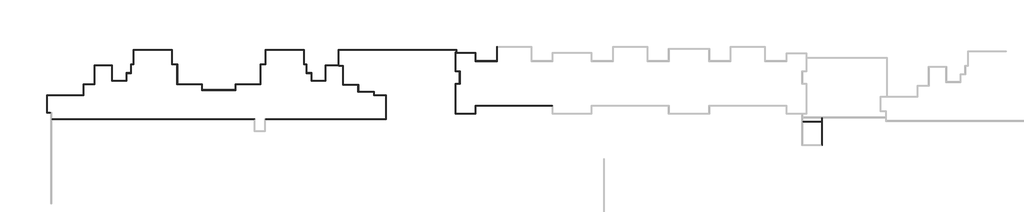
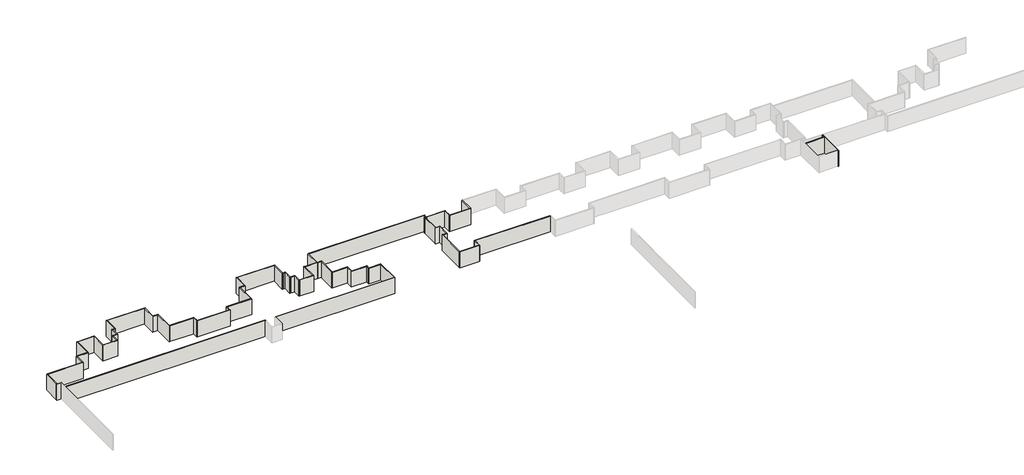
# One storey, part 5 of 8: 63 walls.
"""IFC4 building model written with IfcOpenShell, lengths in millimetres."""

from ifc_helpers import new_model, si_unit, origin, origin_with_axes, place, context, project, spatial, polyline, outline, extrude, faceted_brep, element, save

model = new_model("IFC4")

# Units and contexts
model_context = context("Model", 3, world=origin())
ifc_project = project(units=[si_unit("LENGTHUNIT", "METRE", prefix="MILLI")], contexts=[model_context])

# Site, building, storey
site = spatial("IfcSite", under=ifc_project)
building = spatial("IfcBuilding", under=site)
storey = spatial("IfcBuildingStorey", under=building, Name="户型图", Elevation=0.0)

# Walls
placement = place(None, origin())
element("IfcWall", 1, ObjectType="所有墙体", at=placement, inside=storey, context=model_context, shape_type="Brep", body=[
    faceted_brep([(84990.3013454, 129402.6292795, 0.0), (84259.8101643, 129402.6292795, 0.0), (84139.8101643, 129402.6292795, 0.0), (84139.8101643, 129402.6292795, 3300.0), (84259.8101643, 129402.6292795, 3300.0), (84990.3013454, 129402.6292795, 3300.0), (84990.3013454, 129282.6292795, 0.0), (84990.3013454, 129282.6292795, 3300.0), (84139.8101643, 129282.6292795, 3300.0), (84139.8101643, 129282.6292795, 0.0)], [[[0, 1, 2, 3, 4, 5]], [[6, 7, 8, 9]], [[2, 1, 0, 6, 9]], [[5, 4, 3, 8, 7]], [[0, 5, 7, 6]], [[3, 2, 9, 8]]]),
])
element("IfcWall", 2, ObjectType="所有墙体", at=placement, inside=storey, context=model_context, shape_type="Brep", body=[
    faceted_brep([(84259.8101643, 129402.6292795, 0.0), (84259.8101643, 132682.6292767, 0.0), (84259.8101643, 132802.6292767, 0.0), (84259.8101643, 132802.6292767, 3300.0), (84259.8101643, 132682.6292767, 3300.0), (84259.8101643, 129402.6292795, 3300.0), (84139.8101643, 129402.6292795, 0.0), (84139.8101643, 129402.6292795, 3300.0), (84139.8101643, 132802.6292767, 3300.0), (84139.8101643, 132802.6292767, 0.0)], [[[0, 1, 2, 3, 4, 5]], [[6, 7, 8, 9]], [[2, 1, 0, 6, 9]], [[5, 4, 3, 8, 7]], [[0, 5, 7, 6]], [[3, 2, 9, 8]]]),
])
element("IfcWall", 3, ObjectType="所有墙体", at=placement, inside=storey, context=model_context, shape_type="Brep", body=[
    faceted_brep([(84259.8101643, 132682.6292767, 0.0), (91359.8101643, 132682.6292767, 0.0), (91359.8101643, 132682.6292767, 3300.0), (84259.8101643, 132682.6292767, 3300.0), (84259.8101643, 132802.6292767, 0.0), (84259.8101643, 132802.6292767, 3300.0), (91239.8101643, 132802.6292767, 3300.0), (91359.8101643, 132802.6292767, 3300.0), (91359.8101643, 132802.6292767, 0.0), (91239.8101643, 132802.6292767, 0.0)], [[[0, 1, 2, 3]], [[4, 5, 6, 7, 8, 9]], [[1, 0, 4, 9, 8]], [[3, 2, 7, 6, 5]], [[0, 3, 5, 4]], [[2, 1, 8, 7]]]),
])
element("IfcWall", 4, ObjectType="所有墙体", at=placement, inside=storey, context=model_context, shape_type="Brep", body=[
    faceted_brep([(91359.8101643, 132802.6292767, 0.0), (91359.8101643, 134782.6292766, 0.0), (91359.8101643, 134902.6292766, 0.0), (91359.8101643, 134902.6292766, 3300.0), (91359.8101643, 134782.6292766, 3300.0), (91359.8101643, 132802.6292767, 3300.0), (91239.8101643, 132802.6292767, 0.0), (91239.8101643, 132802.6292767, 3300.0), (91239.8101643, 134902.6292766, 3300.0), (91239.8101643, 134902.6292766, 0.0)], [[[0, 1, 2, 3, 4, 5]], [[6, 7, 8, 9]], [[2, 1, 0, 6, 9]], [[5, 4, 3, 8, 7]], [[0, 5, 7, 6]], [[3, 2, 9, 8]]]),
])
element("IfcWall", 5, ObjectType="所有墙体", at=placement, inside=storey, context=model_context, shape_type="Brep", body=[
    faceted_brep([(91359.8101643, 134782.6292766, 0.0), (93559.8101642, 134782.6292766, 0.0), (93559.8101642, 134782.6292766, 3300.0), (91359.8101643, 134782.6292766, 3300.0), (91359.8101643, 134902.6292766, 0.0), (91359.8101643, 134902.6292766, 3300.0), (93439.8101642, 134902.6292766, 3300.0), (93559.8101642, 134902.6292766, 3300.0), (93559.8101642, 134902.6292766, 0.0), (93439.8101642, 134902.6292766, 0.0)], [[[0, 1, 2, 3]], [[4, 5, 6, 7, 8, 9]], [[1, 0, 4, 9, 8]], [[3, 2, 7, 6, 5]], [[0, 3, 5, 4]], [[2, 1, 8, 7]]]),
])
element("IfcWall", 6, ObjectType="所有墙体", at=placement, inside=storey, context=model_context, shape_type="Brep", body=[
    faceted_brep([(93559.8101642, 134902.6292766, 0.0), (93559.8101642, 138482.6292767, 0.0), (93559.8101642, 138602.6292767, 0.0), (93559.8101642, 138602.6292767, 3300.0), (93559.8101642, 138482.6292767, 3300.0), (93559.8101642, 134902.6292766, 3300.0), (93439.8101642, 134902.6292766, 0.0), (93439.8101642, 134902.6292766, 3300.0), (93439.8101642, 138602.6292767, 3300.0), (93439.8101642, 138602.6292767, 0.0)], [[[0, 1, 2, 3, 4, 5]], [[6, 7, 8, 9]], [[2, 1, 0, 6, 9]], [[5, 4, 3, 8, 7]], [[0, 5, 7, 6]], [[3, 2, 9, 8]]]),
])
element("IfcWall", 7, ObjectType="所有墙体", at=placement, inside=storey, context=model_context, shape_type="Brep", body=[
    faceted_brep([(93559.8101642, 138482.6292767, 0.0), (96839.8101642, 138482.6292767, 0.0), (96959.8101642, 138482.6292767, 0.0), (96959.8101642, 138482.6292767, 3300.0), (96839.8101642, 138482.6292767, 3300.0), (93559.8101642, 138482.6292767, 3300.0), (93559.8101642, 138602.6292767, 0.0), (93559.8101642, 138602.6292767, 3300.0), (96959.8101642, 138602.6292767, 3300.0), (96959.8101642, 138602.6292767, 0.0)], [[[0, 1, 2, 3, 4, 5]], [[6, 7, 8, 9]], [[2, 1, 0, 6, 9]], [[5, 4, 3, 8, 7]], [[0, 5, 7, 6]], [[3, 2, 9, 8]]]),
])
element("IfcWall", 8, ObjectType="所有墙体", at=placement, inside=storey, context=model_context, shape_type="Brep", body=[
    faceted_brep([(96839.8101642, 138482.6292767, 0.0), (96839.8101642, 135482.6292767, 0.0), (96839.8101642, 135482.6292767, 3300.0), (96839.8101642, 138482.6292767, 3300.0), (96959.8101642, 138482.6292767, 0.0), (96959.8101642, 138482.6292767, 3300.0), (96959.8101642, 135602.6292767, 3300.0), (96959.8101642, 135482.6292767, 3300.0), (96959.8101642, 135482.6292767, 0.0), (96959.8101642, 135602.6292767, 0.0)], [[[0, 1, 2, 3]], [[4, 5, 6, 7, 8, 9]], [[1, 0, 4, 9, 8]], [[3, 2, 7, 6, 5]], [[0, 3, 5, 4]], [[2, 1, 8, 7]]]),
])
element("IfcWall", 9, ObjectType="所有墙体", at=placement, inside=storey, context=model_context, shape_type="Brep", body=[
    faceted_brep([(96959.8101642, 135482.6292767, 0.0), (99760.1109232, 135482.6292767, 0.0), (99760.1109232, 135482.6292767, 3300.0), (96959.8101642, 135482.6292767, 3300.0), (96959.8101642, 135602.6292767, 0.0), (96959.8101642, 135602.6292767, 3300.0), (99640.1109232, 135602.6292767, 3300.0), (99760.1109232, 135602.6292767, 3300.0), (99760.1109232, 135602.6292767, 0.0), (99640.1109232, 135602.6292767, 0.0)], [[[0, 1, 2, 3]], [[4, 5, 6, 7, 8, 9]], [[1, 0, 4, 9, 8]], [[3, 2, 7, 6, 5]], [[0, 3, 5, 4]], [[2, 1, 8, 7]]]),
])
element("IfcWall", 10, ObjectType="所有墙体", at=placement, inside=storey, context=model_context, shape_type="Brep", body=[
    faceted_brep([(99760.1109232, 135602.6292767, 0.0), (99760.1109232, 136982.6292752, 0.0), (99760.1109232, 137102.6292752, 0.0), (99760.1109232, 137102.6292752, 3300.0), (99760.1109232, 136982.6292752, 3300.0), (99760.1109232, 135602.6292767, 3300.0), (99640.1109232, 135602.6292767, 0.0), (99640.1109232, 135602.6292767, 3300.0), (99640.1109232, 137102.6292752, 3300.0), (99640.1109232, 137102.6292752, 0.0)], [[[0, 1, 2, 3, 4, 5]], [[6, 7, 8, 9]], [[2, 1, 0, 6, 9]], [[5, 4, 3, 8, 7]], [[0, 5, 7, 6]], [[3, 2, 9, 8]]]),
])
element("IfcWall", 11, ObjectType="所有墙体", at=placement, inside=storey, context=model_context, shape_type="Brep", body=[
    faceted_brep([(99760.1109232, 136982.6292752, 0.0), (100659.8101643, 136982.6292752, 0.0), (100659.8101643, 136982.6292752, 3300.0), (99760.1109232, 136982.6292752, 3300.0), (99760.1109232, 137102.6292752, 0.0), (99760.1109232, 137102.6292752, 3300.0), (100539.8101643, 137102.6292752, 3300.0), (100659.8101643, 137102.6292752, 3300.0), (100659.8101643, 137102.6292752, 0.0), (100539.8101643, 137102.6292752, 0.0)], [[[0, 1, 2, 3]], [[4, 5, 6, 7, 8, 9]], [[1, 0, 4, 9, 8]], [[3, 2, 7, 6, 5]], [[0, 3, 5, 4]], [[2, 1, 8, 7]]]),
])
element("IfcWall", 12, ObjectType="所有墙体", at=placement, inside=storey, context=model_context, shape_type="Brep", body=[
    faceted_brep([(100659.8101643, 137102.6292752, 0.0), (100659.8101643, 138682.6292768, 0.0), (100659.8101643, 138802.6292768, 0.0), (100659.8101643, 138802.6292768, 3300.0), (100659.8101643, 138682.6292768, 3300.0), (100659.8101643, 137102.6292752, 3300.0), (100539.8101643, 137102.6292752, 0.0), (100539.8101643, 137102.6292752, 3300.0), (100539.8101643, 138802.6292768, 3300.0), (100539.8101643, 138802.6292768, 0.0)], [[[0, 1, 2, 3, 4, 5]], [[6, 7, 8, 9]], [[2, 1, 0, 6, 9]], [[5, 4, 3, 8, 7]], [[0, 5, 7, 6]], [[3, 2, 9, 8]]]),
])
element("IfcWall", 13, ObjectType="所有墙体", at=placement, inside=storey, context=model_context, shape_type="Brep", body=[
    faceted_brep([(100659.8101643, 138682.6292768, 0.0), (101159.8101643, 138682.6292768, 0.0), (101159.8101643, 138682.6292768, 3300.0), (100659.8101643, 138682.6292768, 3300.0), (100659.8101643, 138802.6292768, 0.0), (100659.8101643, 138802.6292768, 3300.0), (101039.8101643, 138802.6292768, 3300.0), (101159.8101643, 138802.6292768, 3300.0), (101159.8101643, 138802.6292768, 0.0), (101039.8101643, 138802.6292768, 0.0)], [[[0, 1, 2, 3]], [[4, 5, 6, 7, 8, 9]], [[1, 0, 4, 9, 8]], [[3, 2, 7, 6, 5]], [[0, 3, 5, 4]], [[2, 1, 8, 7]]]),
])
element("IfcWall", 14, ObjectType="所有墙体", at=placement, inside=storey, context=model_context, shape_type="Brep", body=[
    faceted_brep([(101159.8101643, 138802.6292768, 0.0), (101159.8101643, 141482.6292767, 0.0), (101159.8101643, 141602.6292767, 0.0), (101159.8101643, 141602.6292767, 3300.0), (101159.8101643, 141482.6292767, 3300.0), (101159.8101643, 138802.6292768, 3300.0), (101039.8101643, 138802.6292768, 0.0), (101039.8101643, 138802.6292768, 3300.0), (101039.8101643, 141602.6292767, 3300.0), (101039.8101643, 141602.6292767, 0.0)], [[[0, 1, 2, 3, 4, 5]], [[6, 7, 8, 9]], [[2, 1, 0, 6, 9]], [[5, 4, 3, 8, 7]], [[0, 5, 7, 6]], [[3, 2, 9, 8]]]),
])
element("IfcWall", 15, ObjectType="所有墙体", at=placement, inside=storey, context=model_context, shape_type="Brep", body=[
    faceted_brep([(101159.8101643, 141482.6292767, 0.0), (108539.8101642, 141482.6292767, 0.0), (108659.8101642, 141482.6292767, 0.0), (108659.8101642, 141482.6292767, 3300.0), (108539.8101642, 141482.6292767, 3300.0), (101159.8101643, 141482.6292767, 3300.0), (101159.8101643, 141602.6292767, 0.0), (101159.8101643, 141602.6292767, 3300.0), (108659.8101642, 141602.6292767, 3300.0), (108659.8101642, 141602.6292767, 0.0)], [[[0, 1, 2, 3, 4, 5]], [[6, 7, 8, 9]], [[2, 1, 0, 6, 9]], [[5, 4, 3, 8, 7]], [[0, 5, 7, 6]], [[3, 2, 9, 8]]]),
])
element("IfcWall", 16, ObjectType="所有墙体", at=placement, inside=storey, context=model_context, shape_type="Brep", body=[
    faceted_brep([(108539.8101642, 141482.6292767, 0.0), (108539.8101642, 138682.6292768, 0.0), (108539.8101642, 138682.6292768, 3300.0), (108539.8101642, 141482.6292767, 3300.0), (108659.8101642, 141482.6292767, 0.0), (108659.8101642, 141482.6292767, 3300.0), (108659.8101642, 138802.6292768, 3300.0), (108659.8101642, 138682.6292768, 3300.0), (108659.8101642, 138682.6292768, 0.0), (108659.8101642, 138802.6292768, 0.0)], [[[0, 1, 2, 3]], [[4, 5, 6, 7, 8, 9]], [[1, 0, 4, 9, 8]], [[3, 2, 7, 6, 5]], [[0, 3, 5, 4]], [[2, 1, 8, 7]]]),
])
element("IfcWall", 17, ObjectType="所有墙体", at=placement, inside=storey, context=model_context, shape_type="Brep", body=[
    faceted_brep([(108659.8101642, 138682.6292768, 0.0), (109539.8775938, 138682.6292768, 0.0), (109659.8775938, 138682.6292768, 0.0), (109659.8775938, 138682.6292768, 3300.0), (109539.8775938, 138682.6292768, 3300.0), (108659.8101642, 138682.6292768, 3300.0), (108659.8101642, 138802.6292768, 0.0), (108659.8101642, 138802.6292768, 3300.0), (109659.8775938, 138802.6292768, 3300.0), (109659.8775938, 138802.6292768, 0.0)], [[[0, 1, 2, 3, 4, 5]], [[6, 7, 8, 9]], [[2, 1, 0, 6, 9]], [[5, 4, 3, 8, 7]], [[0, 5, 7, 6]], [[3, 2, 9, 8]]]),
])
element("IfcWall", 18, ObjectType="所有墙体", at=placement, inside=storey, context=model_context, shape_type="Brep", body=[
    faceted_brep([(109539.8775938, 138682.6292768, 0.0), (109539.8775938, 134782.6292766, 0.0), (109539.8775938, 134782.6292766, 3300.0), (109539.8775938, 138682.6292768, 3300.0), (109659.8775938, 138682.6292768, 0.0), (109659.8775938, 138682.6292768, 3300.0), (109659.8775938, 134902.6292766, 3300.0), (109659.8775938, 134782.6292766, 3300.0), (109659.8775938, 134782.6292766, 0.0), (109659.8775938, 134902.6292766, 0.0)], [[[0, 1, 2, 3]], [[4, 5, 6, 7, 8, 9]], [[1, 0, 4, 9, 8]], [[3, 2, 7, 6, 5]], [[0, 3, 5, 4]], [[2, 1, 8, 7]]]),
])
element("IfcWall", 19, ObjectType="所有墙体", at=placement, inside=storey, context=model_context, shape_type="Brep", body=[
    faceted_brep([(109659.8775938, 134782.6292766, 0.0), (114389.8101643, 134782.6292766, 0.0), (114509.8101643, 134782.6292766, 0.0), (114509.8101643, 134782.6292766, 3300.0), (114389.8101643, 134782.6292766, 3300.0), (109659.8775938, 134782.6292766, 3300.0), (109659.8775938, 134902.6292766, 0.0), (109659.8775938, 134902.6292766, 3300.0), (114509.8101643, 134902.6292766, 3300.0), (114509.8101643, 134902.6292766, 0.0)], [[[0, 1, 2, 3, 4, 5]], [[6, 7, 8, 9]], [[2, 1, 0, 6, 9]], [[5, 4, 3, 8, 7]], [[0, 5, 7, 6]], [[3, 2, 9, 8]]]),
])
element("IfcWall", 20, ObjectType="所有墙体", at=placement, inside=storey, context=model_context, shape_type="Brep", body=[
    faceted_brep([(114389.8101643, 134782.6292766, 0.0), (114389.8101643, 133682.6292771, 0.0), (114389.8101643, 133682.6292771, 3300.0), (114389.8101643, 134782.6292766, 3300.0), (114509.8101643, 134782.6292766, 0.0), (114509.8101643, 134782.6292766, 3300.0), (114509.8101643, 133802.6292771, 3300.0), (114509.8101643, 133682.6292771, 3300.0), (114509.8101643, 133682.6292771, 0.0), (114509.8101643, 133802.6292771, 0.0)], [[[0, 1, 2, 3]], [[4, 5, 6, 7, 8, 9]], [[1, 0, 4, 9, 8]], [[3, 2, 7, 6, 5]], [[0, 3, 5, 4]], [[2, 1, 8, 7]]]),
])
element("IfcWall", 21, ObjectType="所有墙体", at=placement, inside=storey, context=model_context, shape_type="Brep", body=[
    faceted_brep([(114509.8101643, 133682.6292771, 0.0), (121009.8101642, 133682.6292771, 0.0), (121009.8101642, 133682.6292771, 3300.0), (114509.8101643, 133682.6292771, 3300.0), (114509.8101643, 133802.6292771, 0.0), (114509.8101643, 133802.6292771, 3300.0), (120889.8101642, 133802.6292771, 3300.0), (121009.8101642, 133802.6292771, 3300.0), (121009.8101642, 133802.6292771, 0.0), (120889.8101642, 133802.6292771, 0.0)], [[[0, 1, 2, 3]], [[4, 5, 6, 7, 8, 9]], [[1, 0, 4, 9, 8]], [[3, 2, 7, 6, 5]], [[0, 3, 5, 4]], [[2, 1, 8, 7]]]),
])
element("IfcWall", 22, ObjectType="所有墙体", at=placement, inside=storey, context=model_context, shape_type="Brep", body=[
    faceted_brep([(121009.8101642, 133802.6292771, 0.0), (121009.8101642, 134782.6292766, 0.0), (121009.8101642, 134902.6292766, 0.0), (121009.8101642, 134902.6292766, 3300.0), (121009.8101642, 134782.6292766, 3300.0), (121009.8101642, 133802.6292771, 3300.0), (120889.8101642, 133802.6292771, 0.0), (120889.8101642, 133802.6292771, 3300.0), (120889.8101642, 134902.6292766, 3300.0), (120889.8101642, 134902.6292766, 0.0)], [[[0, 1, 2, 3, 4, 5]], [[6, 7, 8, 9]], [[2, 1, 0, 6, 9]], [[5, 4, 3, 8, 7]], [[0, 5, 7, 6]], [[3, 2, 9, 8]]]),
])
element("IfcWall", 23, ObjectType="所有墙体", at=placement, inside=storey, context=model_context, shape_type="Brep", body=[
    faceted_brep([(121009.8101642, 134782.6292766, 0.0), (125856.9756647, 134782.6292766, 0.0), (125856.9756647, 134782.6292766, 3300.0), (121009.8101642, 134782.6292766, 3300.0), (121009.8101642, 134902.6292766, 0.0), (121009.8101642, 134902.6292766, 3300.0), (125736.9756647, 134902.6292766, 3300.0), (125856.9756647, 134902.6292766, 3300.0), (125856.9756647, 134902.6292766, 0.0), (125736.9756647, 134902.6292766, 0.0)], [[[0, 1, 2, 3]], [[4, 5, 6, 7, 8, 9]], [[1, 0, 4, 9, 8]], [[3, 2, 7, 6, 5]], [[0, 3, 5, 4]], [[2, 1, 8, 7]]]),
])
element("IfcWall", 24, ObjectType="所有墙体", at=placement, inside=storey, context=model_context, shape_type="Brep", body=[
    faceted_brep([(125856.9756647, 134902.6292766, 0.0), (125856.9756647, 138682.6292768, 0.0), (125856.9756647, 138802.6292768, 0.0), (125856.9756647, 138802.6292768, 3300.0), (125856.9756647, 138682.6292768, 3300.0), (125856.9756647, 134902.6292766, 3300.0), (125736.9756647, 134902.6292766, 0.0), (125736.9756647, 134902.6292766, 3300.0), (125736.9756647, 138802.6292768, 3300.0), (125736.9756647, 138802.6292768, 0.0)], [[[0, 1, 2, 3, 4, 5]], [[6, 7, 8, 9]], [[2, 1, 0, 6, 9]], [[5, 4, 3, 8, 7]], [[0, 5, 7, 6]], [[3, 2, 9, 8]]]),
])
element("IfcWall", 25, ObjectType="所有墙体", at=placement, inside=storey, context=model_context, shape_type="Brep", body=[
    faceted_brep([(125856.9756647, 138682.6292768, 0.0), (126856.9756647, 138682.6292768, 0.0), (126856.9756647, 138682.6292768, 3300.0), (125856.9756647, 138682.6292768, 3300.0), (125856.9756647, 138802.6292768, 0.0), (125856.9756647, 138802.6292768, 3300.0), (126736.9756647, 138802.6292768, 3300.0), (126856.9756647, 138802.6292768, 3300.0), (126856.9756647, 138802.6292768, 0.0), (126736.9756647, 138802.6292768, 0.0)], [[[0, 1, 2, 3]], [[4, 5, 6, 7, 8, 9]], [[1, 0, 4, 9, 8]], [[3, 2, 7, 6, 5]], [[0, 3, 5, 4]], [[2, 1, 8, 7]]]),
])
element("IfcWall", 26, ObjectType="所有墙体", at=placement, inside=storey, context=model_context, shape_type="Brep", body=[
    faceted_brep([(126856.9756647, 138802.6292768, 0.0), (126856.9756647, 141482.6292767, 0.0), (126856.9756647, 141602.6292767, 0.0), (126856.9756647, 141602.6292767, 3300.0), (126856.9756647, 141482.6292767, 3300.0), (126856.9756647, 138802.6292768, 3300.0), (126736.9756647, 138802.6292768, 0.0), (126736.9756647, 138802.6292768, 3300.0), (126736.9756647, 141602.6292767, 3300.0), (126736.9756647, 141602.6292767, 0.0)], [[[0, 1, 2, 3, 4, 5]], [[6, 7, 8, 9]], [[2, 1, 0, 6, 9]], [[5, 4, 3, 8, 7]], [[0, 5, 7, 6]], [[3, 2, 9, 8]]]),
])
element("IfcWall", 27, ObjectType="所有墙体", at=placement, inside=storey, context=model_context, shape_type="Brep", body=[
    faceted_brep([(126856.9756647, 141482.6292767, 0.0), (134239.8101637, 141482.6292767, 0.0), (134359.8101637, 141482.6292767, 0.0), (134359.8101637, 141482.6292767, 3300.0), (134239.8101637, 141482.6292767, 3300.0), (126856.9756647, 141482.6292767, 3300.0), (126856.9756647, 141602.6292767, 0.0), (126856.9756647, 141602.6292767, 3300.0), (134359.8101637, 141602.6292767, 3300.0), (134359.8101637, 141602.6292767, 0.0)], [[[0, 1, 2, 3, 4, 5]], [[6, 7, 8, 9]], [[2, 1, 0, 6, 9]], [[5, 4, 3, 8, 7]], [[0, 5, 7, 6]], [[3, 2, 9, 8]]]),
])
element("IfcWall", 28, ObjectType="所有墙体", at=placement, inside=storey, context=model_context, shape_type="Brep", body=[
    faceted_brep([(134239.8101637, 141482.6292767, 0.0), (134239.8101637, 138682.6292768, 0.0), (134239.8101637, 138682.6292768, 3300.0), (134239.8101637, 141482.6292767, 3300.0), (134359.8101637, 141482.6292767, 0.0), (134359.8101637, 141482.6292767, 3300.0), (134359.8101637, 138802.6292768, 3300.0), (134359.8101637, 138682.6292768, 3300.0), (134359.8101637, 138682.6292768, 0.0), (134359.8101637, 138802.6292768, 0.0)], [[[0, 1, 2, 3]], [[4, 5, 6, 7, 8, 9]], [[1, 0, 4, 9, 8]], [[3, 2, 7, 6, 5]], [[0, 3, 5, 4]], [[2, 1, 8, 7]]]),
])
element("IfcWall", 29, ObjectType="所有墙体", at=placement, inside=storey, context=model_context, shape_type="Brep", body=[
    faceted_brep([(134359.8101637, 138682.6292768, 0.0), (134739.8101637, 138682.6292768, 0.0), (134859.8101637, 138682.6292768, 0.0), (134859.8101637, 138682.6292768, 3300.0), (134739.8101637, 138682.6292768, 3300.0), (134359.8101637, 138682.6292768, 3300.0), (134359.8101637, 138802.6292768, 0.0), (134359.8101637, 138802.6292768, 3300.0), (134859.8101637, 138802.6292768, 3300.0), (134859.8101637, 138802.6292768, 0.0)], [[[0, 1, 2, 3, 4, 5]], [[6, 7, 8, 9]], [[2, 1, 0, 6, 9]], [[5, 4, 3, 8, 7]], [[0, 5, 7, 6]], [[3, 2, 9, 8]]]),
])
element("IfcWall", 30, ObjectType="所有墙体", at=placement, inside=storey, context=model_context, shape_type="Brep", body=[
    faceted_brep([(134739.8101637, 138682.6292768, 0.0), (134739.8101637, 136982.6292752, 0.0), (134739.8101637, 136982.6292752, 3300.0), (134739.8101637, 138682.6292768, 3300.0), (134859.8101637, 138682.6292768, 0.0), (134859.8101637, 138682.6292768, 3300.0), (134859.8101637, 137102.6292752, 3300.0), (134859.8101637, 136982.6292752, 3300.0), (134859.8101637, 136982.6292752, 0.0), (134859.8101637, 137102.6292752, 0.0)], [[[0, 1, 2, 3]], [[4, 5, 6, 7, 8, 9]], [[1, 0, 4, 9, 8]], [[3, 2, 7, 6, 5]], [[0, 3, 5, 4]], [[2, 1, 8, 7]]]),
])
element("IfcWall", 31, ObjectType="所有墙体", at=placement, inside=storey, context=model_context, shape_type="Brep", body=[
    faceted_brep([(134859.8101637, 136982.6292752, 0.0), (135639.5094055, 136982.6292752, 0.0), (135759.5094055, 136982.6292752, 0.0), (135759.5094055, 136982.6292752, 3300.0), (135639.5094055, 136982.6292752, 3300.0), (134859.8101637, 136982.6292752, 3300.0), (134859.8101637, 137102.6292752, 0.0), (134859.8101637, 137102.6292752, 3300.0), (135759.5094055, 137102.6292752, 3300.0), (135759.5094055, 137102.6292752, 0.0)], [[[0, 1, 2, 3, 4, 5]], [[6, 7, 8, 9]], [[2, 1, 0, 6, 9]], [[5, 4, 3, 8, 7]], [[0, 5, 7, 6]], [[3, 2, 9, 8]]]),
])
element("IfcWall", 32, ObjectType="所有墙体", at=placement, inside=storey, context=model_context, shape_type="Brep", body=[
    faceted_brep([(135639.5094055, 136982.6292752, 0.0), (135639.5094055, 135482.6292767, 0.0), (135639.5094055, 135482.6292767, 3300.0), (135639.5094055, 136982.6292752, 3300.0), (135759.5094055, 136982.6292752, 0.0), (135759.5094055, 136982.6292752, 3300.0), (135759.5094055, 135602.6292767, 3300.0), (135759.5094055, 135482.6292767, 3300.0), (135759.5094055, 135482.6292767, 0.0), (135759.5094055, 135602.6292767, 0.0)], [[[0, 1, 2, 3]], [[4, 5, 6, 7, 8, 9]], [[1, 0, 4, 9, 8]], [[3, 2, 7, 6, 5]], [[0, 3, 5, 4]], [[2, 1, 8, 7]]]),
])
element("IfcWall", 33, ObjectType="所有墙体", at=placement, inside=storey, context=model_context, shape_type="Brep", body=[
    faceted_brep([(135759.5094055, 135482.6292767, 0.0), (138559.8101637, 135482.6292767, 0.0), (138559.8101637, 135482.6292767, 3300.0), (135759.5094055, 135482.6292767, 3300.0), (135759.5094055, 135602.6292767, 0.0), (135759.5094055, 135602.6292767, 3300.0), (138439.8101637, 135602.6292767, 3300.0), (138559.8101637, 135602.6292767, 3300.0), (138559.8101637, 135602.6292767, 0.0), (138439.8101637, 135602.6292767, 0.0)], [[[0, 1, 2, 3]], [[4, 5, 6, 7, 8, 9]], [[1, 0, 4, 9, 8]], [[3, 2, 7, 6, 5]], [[0, 3, 5, 4]], [[2, 1, 8, 7]]]),
])
element("IfcWall", 34, ObjectType="所有墙体", at=placement, inside=storey, context=model_context, shape_type="Brep", body=[
    faceted_brep([(138559.8101637, 135602.6292767, 0.0), (138559.8101637, 138482.6292767, 0.0), (138559.8101637, 138602.6292767, 0.0), (138559.8101637, 138602.6292767, 3300.0), (138559.8101637, 138482.6292767, 3300.0), (138559.8101637, 135602.6292767, 3300.0), (138439.8101637, 135602.6292767, 0.0), (138439.8101637, 135602.6292767, 3300.0), (138439.8101637, 138602.6292767, 3300.0), (138439.8101637, 138602.6292767, 0.0)], [[[0, 1, 2, 3, 4, 5]], [[6, 7, 8, 9]], [[2, 1, 0, 6, 9]], [[5, 4, 3, 8, 7]], [[0, 5, 7, 6]], [[3, 2, 9, 8]]]),
])
element("IfcWall", 35, ObjectType="所有墙体", at=placement, inside=storey, context=model_context, shape_type="Brep", body=[
    faceted_brep([(138559.8101637, 138482.6292767, 0.0), (141059.8101645, 138482.6292767, 0.0), (141059.8101645, 138482.6292767, 3300.0), (138559.8101637, 138482.6292767, 3300.0), (138559.8101637, 138602.6292767, 0.0), (138559.8101637, 138602.6292767, 3300.0), (140939.8101645, 138602.6292767, 3300.0), (141059.8101645, 138602.6292767, 3300.0), (141059.8101645, 138602.6292767, 0.0), (140939.8101645, 138602.6292767, 0.0), (141059.8101645, 138552.6292795, 0.0), (141059.8101645, 138552.6292795, 3300.0)], [[[0, 1, 2, 3]], [[4, 5, 6, 7, 8, 9]], [[1, 0, 4, 9, 8, 10]], [[3, 2, 11, 7, 6, 5]], [[0, 3, 5, 4]], [[2, 1, 10, 8, 7, 11]]]),
])
element("IfcWall", 36, ObjectType="所有墙体", at=placement, inside=storey, context=model_context, shape_type="Brep", body=[
    faceted_brep([(141059.8101645, 138602.6292767, 0.0), (141059.8101645, 141482.6292767, 0.0), (141059.8101645, 141602.6292767, 0.0), (141059.8101645, 141602.6292767, 3300.0), (141059.8101645, 141482.6292767, 3300.0), (141059.8101645, 138602.6292767, 3300.0), (140939.8101645, 138602.6292767, 0.0), (140939.8101645, 138602.6292767, 3300.0), (140939.8101645, 141602.6292767, 3300.0), (140939.8101645, 141602.6292767, 0.0)], [[[0, 1, 2, 3, 4, 5]], [[6, 7, 8, 9]], [[2, 1, 0, 6, 9]], [[5, 4, 3, 8, 7]], [[0, 5, 7, 6]], [[3, 2, 9, 8]]]),
])
element("IfcWall", 37, ObjectType="所有墙体", at=placement, inside=storey, context=model_context, shape_type="Brep", body=[
    faceted_brep([(141059.8101645, 141482.6292767, 0.0), (163940.6969765, 141482.6292767, 0.0), (164060.6969765, 141482.6292767, 0.0), (164060.6969765, 141482.6292767, 3300.0), (163940.6969765, 141482.6292767, 3300.0), (141059.8101645, 141482.6292767, 3300.0), (141059.8101645, 141602.6292767, 0.0), (141059.8101645, 141602.6292767, 3300.0), (164060.6969765, 141602.6292767, 3300.0), (164060.6969765, 141602.6292767, 0.0)], [[[0, 1, 2, 3, 4, 5]], [[6, 7, 8, 9]], [[2, 1, 0, 6, 9]], [[5, 4, 3, 8, 7]], [[0, 5, 7, 6]], [[3, 2, 9, 8]]]),
])
element("IfcWall", 38, ObjectType="所有墙体", at=placement, inside=storey, context=model_context, shape_type="Brep", body=[
    faceted_brep([(163940.6969765, 141482.6292767, 0.0), (163940.6969765, 141102.629274, 0.0), (163940.6969765, 140982.629274, 0.0), (163940.6969765, 140905.0802708, 0.0), (163940.6969765, 140905.0802708, 3300.0), (163940.6969765, 140982.629274, 3300.0), (163940.6969765, 141102.629274, 3300.0), (163940.6969765, 141482.6292767, 3300.0), (164060.6969765, 141482.6292767, 0.0), (164060.6969765, 141482.6292767, 3300.0), (164060.6969765, 141025.0802708, 3300.0), (164060.6969765, 140905.0802708, 3300.0), (164060.6969765, 140905.0802708, 0.0), (164060.6969765, 141025.0802708, 0.0)], [[[0, 1, 2, 3, 4, 5, 6, 7]], [[8, 9, 10, 11, 12, 13]], [[3, 2, 1, 0, 8, 13, 12]], [[7, 6, 5, 4, 11, 10, 9]], [[0, 7, 9, 8]], [[4, 3, 12, 11]]]),
])
element("IfcWall", 39, ObjectType="所有墙体", at=placement, inside=storey, context=model_context, shape_type="Brep", body=[
    faceted_brep([(164060.6969765, 140905.0802708, 0.0), (167640.6969649, 140905.0802708, 0.0), (167760.6969649, 140905.0802708, 0.0), (167760.6969649, 140905.0802708, 3300.0), (167640.6969649, 140905.0802708, 3300.0), (164060.6969765, 140905.0802708, 3300.0), (164060.6969765, 141025.0802708, 0.0), (164060.6969765, 141025.0802708, 3300.0), (167760.6969649, 141025.0802708, 3300.0), (167760.6969649, 141025.0802708, 0.0)], [[[0, 1, 2, 3, 4, 5]], [[6, 7, 8, 9]], [[2, 1, 0, 6, 9]], [[5, 4, 3, 8, 7]], [[0, 5, 7, 6]], [[3, 2, 9, 8]]]),
])
element("IfcWall", 40, ObjectType="所有墙体", at=placement, inside=storey, context=model_context, shape_type="Brep", body=[
    faceted_brep([(167640.6969649, 140905.0802708, 0.0), (167640.6969649, 139327.5312675, 0.0), (167640.6969649, 139327.5312675, 3300.0), (167640.6969649, 140905.0802708, 3300.0), (167760.6969649, 140905.0802708, 0.0), (167760.6969649, 140905.0802708, 3300.0), (167760.6969649, 139447.5312675, 3300.0), (167760.6969649, 139327.5312675, 3300.0), (167760.6969649, 139327.5312675, 0.0), (167760.6969649, 139447.5312675, 0.0)], [[[0, 1, 2, 3]], [[4, 5, 6, 7, 8, 9]], [[1, 0, 4, 9, 8]], [[3, 2, 7, 6, 5]], [[0, 3, 5, 4]], [[2, 1, 8, 7]]]),
])
element("IfcWall", 41, ObjectType="所有墙体", at=placement, inside=storey, context=model_context, shape_type="Brep", body=[
    faceted_brep([(167760.6969649, 139327.5312675, 0.0), (171910.6969649, 139327.5312675, 0.0), (171910.6969649, 139327.5312675, 3300.0), (167760.6969649, 139327.5312675, 3300.0), (167760.6969649, 139447.5312675, 0.0), (167760.6969649, 139447.5312675, 3300.0), (171790.6969649, 139447.5312675, 3300.0), (171910.6969649, 139447.5312675, 3300.0), (171910.6969649, 139447.5312675, 0.0), (171790.6969649, 139447.5312675, 0.0)], [[[0, 1, 2, 3]], [[4, 5, 6, 7, 8, 9]], [[1, 0, 4, 9, 8]], [[3, 2, 7, 6, 5]], [[0, 3, 5, 4]], [[2, 1, 8, 7]]]),
])
element("IfcWall", 42, ObjectType="所有墙体", at=placement, inside=storey, context=model_context, shape_type="Brep", body=[
    faceted_brep([(171910.6969649, 139447.5312675, 0.0), (171910.6969649, 142127.5312689, 0.0), (171910.6969649, 142247.5312689, 0.0), (171910.6969649, 142247.5312689, 3300.0), (171910.6969649, 142127.5312689, 3300.0), (171910.6969649, 139447.5312675, 3300.0), (171790.6969649, 139447.5312675, 0.0), (171790.6969649, 139447.5312675, 3300.0), (171790.6969649, 142247.5312689, 3300.0), (171790.6969649, 142247.5312689, 0.0)], [[[0, 1, 2, 3, 4, 5]], [[6, 7, 8, 9]], [[2, 1, 0, 6, 9]], [[5, 4, 3, 8, 7]], [[0, 5, 7, 6]], [[3, 2, 9, 8]]]),
])
element("IfcWall", 43, ObjectType="所有墙体", at=placement, inside=storey, context=model_context, shape_type="Brep", body=[
    faceted_brep([(182640.6969646, 130747.5312684, 0.0), (167640.6969649, 130747.5312684, 0.0), (167640.6969649, 130747.5312684, 3300.0), (182640.6969646, 130747.5312684, 3300.0), (182640.6969646, 130627.5312684, 0.0), (182640.6969646, 130627.5312684, 3300.0), (167760.6969649, 130627.5312684, 3300.0), (167640.6969649, 130627.5312684, 3300.0), (167640.6969649, 130627.5312684, 0.0), (167760.6969649, 130627.5312684, 0.0)], [[[0, 1, 2, 3]], [[4, 5, 6, 7, 8, 9]], [[1, 0, 4, 9, 8]], [[3, 2, 7, 6, 5]], [[0, 3, 5, 4]], [[2, 1, 8, 7]]]),
])
element("IfcWall", 44, ObjectType="所有墙体", at=placement, inside=storey, context=model_context, shape_type="Brep", body=[
    faceted_brep([(167640.6969649, 130627.5312684, 0.0), (167640.6969649, 129147.5312684, 0.0), (167640.6969649, 129027.5312684, 0.0), (167640.6969649, 129027.5312684, 3300.0), (167640.6969649, 129147.5312684, 3300.0), (167640.6969649, 130627.5312684, 3300.0), (167760.6969649, 130627.5312684, 0.0), (167760.6969649, 130627.5312684, 3300.0), (167760.6969649, 129027.5312684, 3300.0), (167760.6969649, 129027.5312684, 0.0)], [[[0, 1, 2, 3, 4, 5]], [[6, 7, 8, 9]], [[2, 1, 0, 6, 9]], [[5, 4, 3, 8, 7]], [[0, 5, 7, 6]], [[3, 2, 9, 8]]]),
])
element("IfcWall", 45, ObjectType="所有墙体", at=placement, inside=storey, context=model_context, shape_type="Brep", body=[
    faceted_brep([(167640.6969649, 129147.5312684, 0.0), (163860.6969648, 129147.5312684, 0.0), (163740.6969648, 129147.5312684, 0.0), (163740.6969648, 129147.5312684, 3300.0), (163860.6969648, 129147.5312684, 3300.0), (167640.6969649, 129147.5312684, 3300.0), (167640.6969649, 129027.5312684, 0.0), (167640.6969649, 129027.5312684, 3300.0), (163740.6969648, 129027.5312684, 3300.0), (163740.6969648, 129027.5312684, 0.0)], [[[0, 1, 2, 3, 4, 5]], [[6, 7, 8, 9]], [[2, 1, 0, 6, 9]], [[5, 4, 3, 8, 7]], [[0, 5, 7, 6]], [[3, 2, 9, 8]]]),
])
element("IfcWall", 46, ObjectType="所有墙体", at=placement, inside=storey, context=model_context, shape_type="Brep", body=[
    faceted_brep([(163860.6969648, 129147.5312684, 0.0), (163860.6969648, 134927.5312611, 0.0), (163860.6969648, 135047.5312611, 0.0), (163860.6969648, 135047.5312611, 3300.0), (163860.6969648, 134927.5312611, 3300.0), (163860.6969648, 129147.5312684, 3300.0), (163740.6969648, 129147.5312684, 0.0), (163740.6969648, 129147.5312684, 3300.0), (163740.6969648, 135047.5312611, 3300.0), (163740.6969648, 135047.5312611, 0.0)], [[[0, 1, 2, 3, 4, 5]], [[6, 7, 8, 9]], [[2, 1, 0, 6, 9]], [[5, 4, 3, 8, 7]], [[0, 5, 7, 6]], [[3, 2, 9, 8]]]),
])
element("IfcWall", 47, ObjectType="所有墙体", at=placement, inside=storey, context=model_context, shape_type="Brep", body=[
    faceted_brep([(163860.6969648, 134927.5312611, 0.0), (164660.6969648, 134927.5312611, 0.0), (164660.6969648, 134927.5312611, 3300.0), (163860.6969648, 134927.5312611, 3300.0), (163860.6969648, 135047.5312611, 0.0), (163860.6969648, 135047.5312611, 3300.0), (164540.6969648, 135047.5312611, 3300.0), (164660.6969648, 135047.5312611, 3300.0), (164660.6969648, 135047.5312611, 0.0), (164540.6969648, 135047.5312611, 0.0)], [[[0, 1, 2, 3]], [[4, 5, 6, 7, 8, 9]], [[1, 0, 4, 9, 8]], [[3, 2, 7, 6, 5]], [[0, 3, 5, 4]], [[2, 1, 8, 7]]]),
])
element("IfcWall", 48, ObjectType="所有墙体", at=placement, inside=storey, context=model_context, shape_type="Brep", body=[
    faceted_brep([(164660.6969648, 135047.5312611, 0.0), (164660.6969648, 137447.5312688, 0.0), (164660.6969648, 137447.5312688, 3300.0), (164660.6969648, 135047.5312611, 3300.0), (164540.6969648, 135047.5312611, 0.0), (164540.6969648, 135047.5312611, 3300.0), (164540.6969648, 137327.5312688, 3300.0), (164540.6969648, 137447.5312688, 3300.0), (164540.6969648, 137447.5312688, 0.0), (164540.6969648, 137327.5312688, 0.0)], [[[0, 1, 2, 3]], [[4, 5, 6, 7, 8, 9]], [[1, 0, 4, 9, 8]], [[3, 2, 7, 6, 5]], [[0, 3, 5, 4]], [[2, 1, 8, 7]]]),
])
element("IfcWall", 49, ObjectType="所有墙体", at=placement, inside=storey, context=model_context, shape_type="Brep", body=[
    faceted_brep([(164540.6969648, 137447.5312688, 0.0), (163860.6969648, 137447.5312688, 0.0), (163740.6969648, 137447.5312688, 0.0), (163740.6969648, 137447.5312688, 3300.0), (163860.6969648, 137447.5312688, 3300.0), (164540.6969648, 137447.5312688, 3300.0), (164540.6969648, 137327.5312688, 0.0), (164540.6969648, 137327.5312688, 3300.0), (163740.6969648, 137327.5312688, 3300.0), (163740.6969648, 137327.5312688, 0.0)], [[[0, 1, 2, 3, 4, 5]], [[6, 7, 8, 9]], [[2, 1, 0, 6, 9]], [[5, 4, 3, 8, 7]], [[0, 5, 7, 6]], [[3, 2, 9, 8]]]),
])
element("IfcWall", 50, ObjectType="所有墙体", at=placement, inside=storey, context=model_context, shape_type="SweptSolid", body=[
    extrude(outline(polyline([(163860.6969648, 140982.629274), (163860.6969648, 137447.5312688), (163740.6969648, 137447.5312688), (163740.6969648, 140982.629274), (163860.6969648, 140982.629274)])), origin_with_axes(), (0.0, 0.0, 1.0), 3300.0),
])
element("IfcWall", 51, ObjectType="所有墙体", at=placement, inside=storey, context=model_context, shape_type="Brep", body=[
    faceted_brep([(163740.6969648, 140982.629274, 0.0), (163860.6969648, 140982.629274, 0.0), (163940.6969765, 140982.629274, 0.0), (163940.6969765, 140982.629274, 3300.0), (163860.6969648, 140982.629274, 3300.0), (163740.6969648, 140982.629274, 3300.0), (163740.6969648, 141102.629274, 0.0), (163740.6969648, 141102.629274, 3300.0), (163940.6969765, 141102.629274, 3300.0), (163940.6969765, 141102.629274, 0.0)], [[[0, 1, 2, 3, 4, 5]], [[6, 7, 8, 9]], [[2, 1, 0, 6, 9]], [[5, 4, 3, 8, 7]], [[0, 5, 7, 6]], [[3, 2, 9, 8]]]),
])
element("IfcWall", 52, ObjectType="所有墙体", at=placement, inside=storey, context=model_context, shape_type="Brep", body=[
    faceted_brep([(85110.3013454, 127947.6292793, 0.0), (124590.5968759, 127947.6292793, 0.0), (124710.5968759, 127947.6292793, 0.0), (124710.5968759, 127947.6292793, 3300.0), (124590.5968759, 127947.6292793, 3300.0), (85110.3013454, 127947.6292793, 3300.0), (85110.3013454, 128067.6292793, 0.0), (85110.3013454, 128067.6292793, 3300.0), (124710.5968759, 128067.6292793, 3300.0), (124710.5968759, 128067.6292793, 0.0)], [[[0, 1, 2, 3, 4, 5]], [[6, 7, 8, 9]], [[2, 1, 0, 6, 9]], [[5, 4, 3, 8, 7]], [[0, 5, 7, 6]], [[3, 2, 9, 8]]]),
])
element("IfcWall", 53, ObjectType="所有墙体", at=placement, inside=storey, context=model_context, shape_type="Brep", body=[
    faceted_brep([(126709.8101643, 127947.6292793, 0.0), (150309.8101643, 127947.6292793, 0.0), (150309.8101643, 127947.6292793, 3300.0), (126709.8101643, 127947.6292793, 3300.0), (126709.8101643, 128067.6292793, 0.0), (126709.8101643, 128067.6292793, 3300.0), (150189.8101643, 128067.6292793, 3300.0), (150309.8101643, 128067.6292793, 3300.0), (150309.8101643, 128067.6292793, 0.0), (150189.8101643, 128067.6292793, 0.0)], [[[0, 1, 2, 3]], [[4, 5, 6, 7, 8, 9]], [[1, 0, 4, 9, 8]], [[3, 2, 7, 6, 5]], [[0, 3, 5, 4]], [[2, 1, 8, 7]]]),
])
element("IfcWall", 54, ObjectType="所有墙体", at=placement, inside=storey, context=model_context, shape_type="Brep", body=[
    faceted_brep([(150309.8101643, 128067.6292793, 0.0), (150309.8101643, 132752.6292796, 0.0), (150309.8101643, 132752.6292796, 3300.0), (150309.8101643, 128067.6292793, 3300.0), (150189.8101643, 128067.6292793, 0.0), (150189.8101643, 128067.6292793, 3300.0), (150189.8101643, 132632.6292796, 3300.0), (150189.8101643, 132752.6292796, 3300.0), (150189.8101643, 132752.6292796, 0.0), (150189.8101643, 132632.6292796, 0.0)], [[[0, 1, 2, 3]], [[4, 5, 6, 7, 8, 9]], [[1, 0, 4, 9, 8]], [[3, 2, 7, 6, 5]], [[0, 3, 5, 4]], [[2, 1, 8, 7]]]),
])
element("IfcWall", 55, ObjectType="所有墙体", at=placement, inside=storey, context=model_context, shape_type="Brep", body=[
    faceted_brep([(150189.8101643, 132752.6292796, 0.0), (147933.8101639, 132752.6292796, 0.0), (147813.8101639, 132752.6292796, 0.0), (147813.8101639, 132752.6292796, 3300.0), (147933.8101639, 132752.6292796, 3300.0), (150189.8101643, 132752.6292796, 3300.0), (150189.8101643, 132632.6292796, 0.0), (150189.8101643, 132632.6292796, 3300.0), (147813.8101639, 132632.6292796, 3300.0), (147813.8101639, 132632.6292796, 0.0)], [[[0, 1, 2, 3, 4, 5]], [[6, 7, 8, 9]], [[2, 1, 0, 6, 9]], [[5, 4, 3, 8, 7]], [[0, 5, 7, 6]], [[3, 2, 9, 8]]]),
])
element("IfcWall", 56, ObjectType="所有墙体", at=placement, inside=storey, context=model_context, shape_type="Brep", body=[
    faceted_brep([(147933.8101639, 132752.6292796, 0.0), (147933.8101639, 133452.6274413, 0.0), (147933.8101639, 133452.6274413, 3300.0), (147933.8101639, 132752.6292796, 3300.0), (147813.8101639, 132752.6292796, 0.0), (147813.8101639, 132752.6292796, 3300.0), (147813.8101639, 133332.6274413, 3300.0), (147813.8101639, 133452.6274413, 3300.0), (147813.8101639, 133452.6274413, 0.0), (147813.8101639, 133332.6274413, 0.0)], [[[0, 1, 2, 3]], [[4, 5, 6, 7, 8, 9]], [[1, 0, 4, 9, 8]], [[3, 2, 7, 6, 5]], [[0, 3, 5, 4]], [[2, 1, 8, 7]]]),
])
element("IfcWall", 57, ObjectType="所有墙体", at=placement, inside=storey, context=model_context, shape_type="Brep", body=[
    faceted_brep([(147813.8101639, 133452.6274413, 0.0), (144909.8101644, 133452.6274413, 0.0), (144789.8101644, 133452.6274413, 0.0), (144789.8101644, 133452.6274413, 3300.0), (144909.8101644, 133452.6274413, 3300.0), (147813.8101639, 133452.6274413, 3300.0), (147813.8101639, 133332.6274413, 0.0), (147813.8101639, 133332.6274413, 3300.0), (144789.8101644, 133332.6274413, 3300.0), (144789.8101644, 133332.6274413, 0.0)], [[[0, 1, 2, 3, 4, 5]], [[6, 7, 8, 9]], [[2, 1, 0, 6, 9]], [[5, 4, 3, 8, 7]], [[0, 5, 7, 6]], [[3, 2, 9, 8]]]),
])
element("IfcWall", 58, ObjectType="所有墙体", at=placement, inside=storey, context=model_context, shape_type="Brep", body=[
    faceted_brep([(144909.8101644, 133452.6274413, 0.0), (144909.8101644, 134842.6292765, 0.0), (144909.8101644, 134842.6292765, 3300.0), (144909.8101644, 133452.6274413, 3300.0), (144789.8101644, 133452.6274413, 0.0), (144789.8101644, 133452.6274413, 3300.0), (144789.8101644, 134722.6292765, 3300.0), (144789.8101644, 134842.6292765, 3300.0), (144789.8101644, 134842.6292765, 0.0), (144789.8101644, 134722.6292765, 0.0)], [[[0, 1, 2, 3]], [[4, 5, 6, 7, 8, 9]], [[1, 0, 4, 9, 8]], [[3, 2, 7, 6, 5]], [[0, 3, 5, 4]], [[2, 1, 8, 7]]]),
])
element("IfcWall", 59, ObjectType="所有墙体", at=placement, inside=storey, context=model_context, shape_type="Brep", body=[
    faceted_brep([(144789.8101644, 134842.6292765, 0.0), (141909.810179, 134842.6292765, 0.0), (141789.810179, 134842.6292765, 0.0), (141789.810179, 134842.6292765, 3300.0), (141909.810179, 134842.6292765, 3300.0), (144789.8101644, 134842.6292765, 3300.0), (144789.8101644, 134722.6292765, 0.0), (144789.8101644, 134722.6292765, 3300.0), (141789.810179, 134722.6292765, 3300.0), (141789.810179, 134722.6292765, 0.0)], [[[0, 1, 2, 3, 4, 5]], [[6, 7, 8, 9]], [[2, 1, 0, 6, 9]], [[5, 4, 3, 8, 7]], [[0, 5, 7, 6]], [[3, 2, 9, 8]]]),
])
element("IfcWall", 60, ObjectType="所有墙体", at=placement, inside=storey, context=model_context, shape_type="Brep", body=[
    faceted_brep([(141909.810179, 134842.6292765, 0.0), (141909.810179, 138552.6292795, 0.0), (141909.810179, 138552.6292795, 3300.0), (141909.810179, 134842.6292765, 3300.0), (141789.810179, 134842.6292765, 0.0), (141789.810179, 134842.6292765, 3300.0), (141789.810179, 138432.6292795, 3300.0), (141789.810179, 138552.6292795, 3300.0), (141789.810179, 138552.6292795, 0.0), (141789.810179, 138432.6292795, 0.0)], [[[0, 1, 2, 3]], [[4, 5, 6, 7, 8, 9]], [[1, 0, 4, 9, 8]], [[3, 2, 7, 6, 5]], [[0, 3, 5, 4]], [[2, 1, 8, 7]]]),
])
element("IfcWall", 61, ObjectType="所有墙体", at=placement, inside=storey, context=model_context, shape_type="Brep", body=[
    faceted_brep([(141789.810179, 138552.6292795, 0.0), (141059.8101645, 138552.6292795, 0.0), (141059.8101645, 138552.6292795, 3300.0), (141789.810179, 138552.6292795, 3300.0), (141789.810179, 138432.6292795, 0.0), (141789.810179, 138432.6292795, 3300.0), (141059.8101645, 138432.6292795, 3300.0), (141059.8101645, 138432.6292795, 0.0), (141059.8101645, 138482.6292767, 0.0), (141059.8101645, 138482.6292767, 3300.0)], [[[0, 1, 2, 3]], [[4, 5, 6, 7]], [[1, 0, 4, 7, 8]], [[3, 2, 9, 6, 5]], [[0, 3, 5, 4]], [[2, 1, 8, 7, 6, 9]]]),
])
element("IfcWall", 62, ObjectType="所有墙体", at=placement, inside=storey, context=model_context, shape_type="Brep", body=[
    faceted_brep([(235089.8041277, 128327.7400891, 0.0), (235089.8041277, 127647.7400892, 0.0), (235089.8041277, 127527.7400892, 0.0), (235089.8041277, 123051.6486698, 0.0), (235089.8041277, 122931.6486698, 0.0), (235089.8041277, 122892.3894162, 0.0), (235089.8041277, 122892.3894162, 2700.0), (235089.8041277, 122892.3894162, 3300.0), (235089.8041277, 122931.6486698, 3300.0), (235089.8041277, 123051.6486698, 3300.0), (235089.8041277, 123192.3894162, 3300.0), (235089.8041277, 127527.7400892, 3300.0), (235089.8041277, 127647.7400892, 3300.0), (235089.8041277, 128327.7400891, 3300.0), (235209.8041277, 128327.7400891, 0.0), (235209.8041277, 128327.7400891, 2700.0), (235209.8041277, 128327.7400891, 3300.0), (235209.8041277, 123192.3894162, 3300.0), (235209.8041277, 122892.3894162, 3300.0), (235209.8041277, 122892.3894162, 2700.0), (235209.8041277, 122892.3894162, 0.0), (235149.8041274, 122892.3894162, 3300.0)], [[[0, 1, 2, 3, 4, 5, 6, 7, 8, 9, 10, 11, 12, 13]], [[14, 15, 16, 17, 18, 19, 20]], [[5, 4, 3, 2, 1, 0, 14, 20]], [[7, 6, 5, 20, 19, 18, 21]], [[13, 12, 11, 10, 9, 8, 7, 21, 18, 17, 16]], [[0, 13, 16, 15, 14]]]),
])
element("IfcWall", 63, ObjectType="所有墙体", at=placement, inside=storey, context=model_context, shape_type="SweptSolid", body=[
    extrude(outline(polyline([(235089.8041277, 127527.7400892), (231369.8041277, 127527.7400892), (231369.8041277, 127647.7400892), (235089.8041277, 127647.7400892), (235089.8041277, 127527.7400892)])), origin_with_axes(), (0.0, 0.0, 1.0), 3300.0),
])

save(model, "model.ifc")

# Revit data of these elements
# Type "所有墙体"
#   Layers, outside or top first: 120 mm "默认" (function 1)
# Elements 1, 2, 3, 4, 5, 6, 7, 8, 9, 10, 11, 12, 13, 14, 15, 16, 17, 18, 19, 20, 21, 22, 23, 24, 25, 26, 27, 28, 29, 30, 31, 32, 33, 34, 35, 36, 37, 38, 39, 40, 41, 42, 43, 44, 45, 46, 47, 48, 49, 50, 51, 52, 53, 54, 55, 56, 57, 58, 59, 60, 61, 62, 63 (IfcWall, "所有墙体")
#   Comments = ""
#   Top Offset = 0 mm
#   Base Offset = 0 mm
#   wall height = 3300 mm
#   Phase Created = 新构造
#   Base Constraint = 户型图
#   Top Constraint = 层高
#   Materials on its faces: "默认"
# Materials
#   "默认": class "其他", colour RGB 192 192 192, transparency 0, Cost = 0
